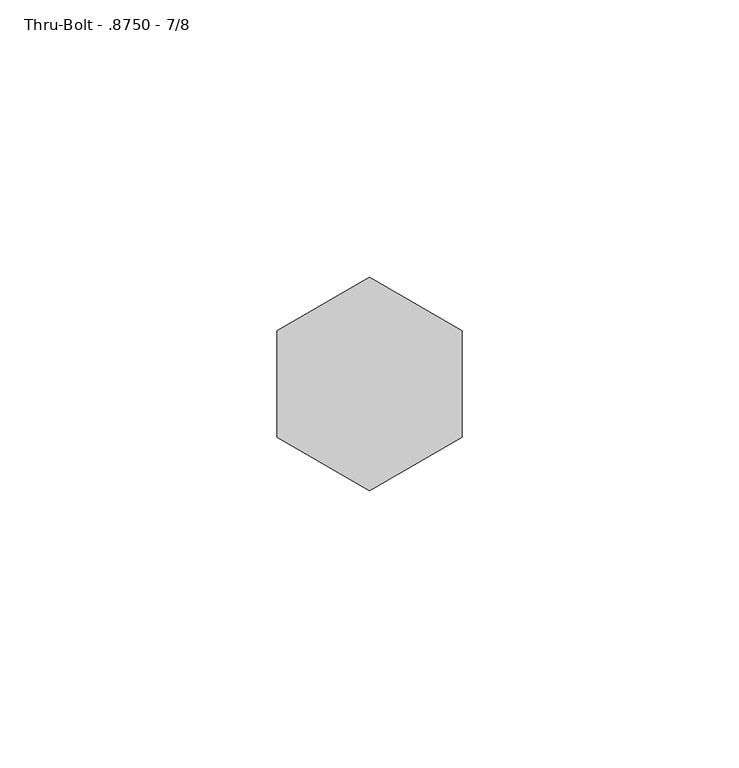
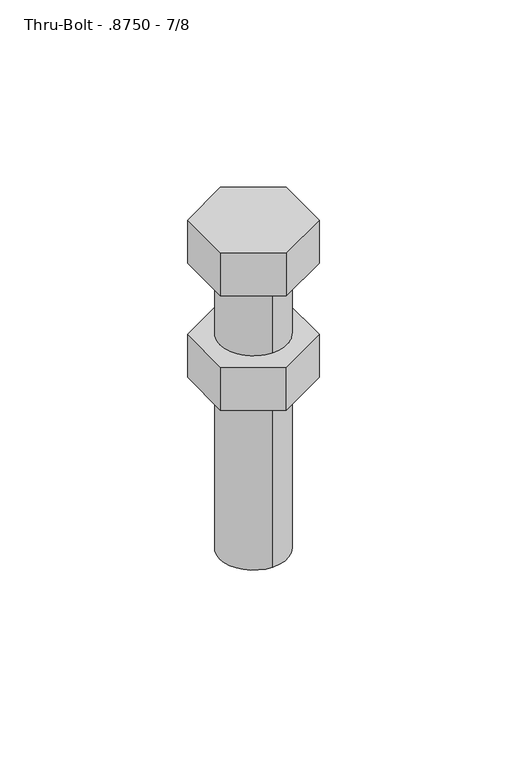
"""IFC4 building model written with IfcOpenShell, lengths in millimetres: fastener geometry, 060523 - W_P_C - Fastenings - Generic : Thru-Bolt - .8750 - 7/8."""

import ifcopenshell
import ifcopenshell.guid

model = None  # the IFC model being written
_history = None  # IfcOwnerHistory: only IFC2X3 demands one
_inside = {}  # id of a spatial element -> (the spatial element, [elements in it])
_under = {}  # id of a project, library or spatial element -> (it, [spatial elements below it])
_declared = {}  # id of a project -> (the project, [libraries it declares])
_typed = {}  # id of a type object -> (the type object, [elements of that type])
_made_of = {}  # id of a material, layer set ... -> (it, [elements and type objects made of it])


def new_model(schema):
    """Start an empty IFC model of exactly this schema.

    Asked for "IFC4X3", IfcOpenShell would pick the latest addendum, in which some entities
    have other attributes; the version numbers below select the first issue.
    IFC2X3 requires an IfcOwnerHistory on every rooted entity: one is made here for all.
    """
    global model, _history
    if schema == "IFC4X3":
        model = ifcopenshell.file(schema_version=(4, 3, 0, 0))
    else:
        model = ifcopenshell.file(schema=schema)
    _inside.clear()
    _under.clear()
    _declared.clear()
    _typed.clear()
    _made_of.clear()
    _history = None
    if model.schema == "IFC2X3":
        org = make("IfcOrganization", Name="unknown")
        user = make(
            "IfcPersonAndOrganization",
            ThePerson=make("IfcPerson", FamilyName="unknown"),
            TheOrganization=org,
        )
        app = make(
            "IfcApplication",
            ApplicationDeveloper=org,
            Version="unknown",
            ApplicationFullName="unknown",
            ApplicationIdentifier="unknown",
        )
        _history = make(
            "IfcOwnerHistory",
            OwningUser=user,
            OwningApplication=app,
            ChangeAction="ADDED",
            CreationDate=0,
        )
    return model


def make(cls, **values):
    """One entity of the class cls with the attributes given. An attribute that is None is left unset."""
    return model.create_entity(
        cls, **{name: value for name, value in values.items() if value is not None}
    )


def rooted(cls, **values):
    """An entity with a GlobalId (a new one), such as an element, a storey or a relation."""
    return make(cls, GlobalId=ifcopenshell.guid.new(), OwnerHistory=_history, **values)


def si_unit(unit_type, name, prefix=None):
    """IfcSIUnit, for example si_unit("LENGTHUNIT", "METRE", prefix="MILLI")."""
    return make("IfcSIUnit", UnitType=unit_type, Prefix=prefix, Name=name)


def assignment(units):
    """IfcUnitAssignment: the units of a project."""
    return None if units is None else make("IfcUnitAssignment", Units=units)


def point(xyz):
    """IfcCartesianPoint."""
    return None if xyz is None else make("IfcCartesianPoint", Coordinates=xyz)


def direction(xyz):
    """IfcDirection."""
    return None if xyz is None else make("IfcDirection", DirectionRatios=xyz)


def frame(location, z_axis=None, x_axis=None):
    """IfcAxis2Placement3D, a coordinate frame: its origin and axes. An axis left out is left unset."""
    return make(
        "IfcAxis2Placement3D",
        Location=point(location),
        Axis=direction(z_axis),
        RefDirection=direction(x_axis),
    )


def frame_2d(location, x_axis=None):
    """IfcAxis2Placement2D, a coordinate frame in the plane: its origin and x axis."""
    return make(
        "IfcAxis2Placement2D", Location=point(location), RefDirection=direction(x_axis)
    )


def origin():
    """The frame at (0, 0, 0) with its axes left unset."""
    return frame((0.0, 0.0, 0.0))


def origin_with_axes():
    """The frame at (0, 0, 0) with the z axis (0, 0, 1) and the x axis (1, 0, 0) written out."""
    return frame((0.0, 0.0, 0.0), z_axis=(0.0, 0.0, 1.0), x_axis=(1.0, 0.0, 0.0))


def origin_2d():
    """The frame at (0, 0) in the plane with its x axis left unset."""
    return frame_2d((0.0, 0.0))


def place(relative_to, where):
    """IfcLocalPlacement: puts the frame where relative to a parent placement (None: the world)."""
    return make(
        "IfcLocalPlacement", PlacementRelTo=relative_to, RelativePlacement=where
    )


def context(
    kind, dimensions, precision=None, world=None, true_north=None, identifier=None
):
    """IfcGeometricRepresentationContext, for example the 3D "Model" context."""
    return make(
        "IfcGeometricRepresentationContext",
        ContextIdentifier=identifier,
        ContextType=kind,
        CoordinateSpaceDimension=dimensions,
        Precision=precision,
        WorldCoordinateSystem=world,
        TrueNorth=true_north,
    )


def project(units=None, contexts=None):
    """IfcProject with its units and contexts."""
    return rooted(
        "IfcProject",
        Name="project",
        RepresentationContexts=contexts,
        UnitsInContext=assignment(units),
    )


def spatial(cls, under=None, at=None, **own):
    """A site, building, storey or space (cls), placed at a placement, below another one or the project."""
    s = rooted(cls, ObjectPlacement=at, **own)
    if under is not None:
        _under.setdefault(under.id(), (under, []))[1].append(s)
    return s


def polyline(points):
    """IfcPolyline through the points."""
    return make("IfcPolyline", Points=[point(p) for p in points])


def circle_curve(where, radius):
    """IfcCircle in the frame where."""
    return make("IfcCircle", Position=where, Radius=radius)


def trimmed(basis, trim1, trim2, sense, master):
    """IfcTrimmedCurve: the piece of a basis curve between two trims."""
    return make(
        "IfcTrimmedCurve",
        BasisCurve=basis,
        Trim1=trim1,
        Trim2=trim2,
        SenseAgreement=sense,
        MasterRepresentation=master,
    )


def segment(curve, same_sense, transition):
    """IfcCompositeCurveSegment."""
    return make(
        "IfcCompositeCurveSegment",
        Transition=transition,
        SameSense=same_sense,
        ParentCurve=curve,
    )


def composite_curve(segments, self_intersect=None):
    """IfcCompositeCurve: segments joined end to end."""
    return make("IfcCompositeCurve", Segments=segments, SelfIntersect=self_intersect)


def outline(outer, holes=None, kind="AREA"):
    """IfcArbitraryClosedProfileDef: a profile drawn as a closed curve; with holes, ...WithVoids."""
    if holes is None:
        return make("IfcArbitraryClosedProfileDef", ProfileType=kind, OuterCurve=outer)
    return make(
        "IfcArbitraryProfileDefWithVoids",
        ProfileType=kind,
        OuterCurve=outer,
        InnerCurves=holes,
    )


def extrude(swept, where, along, depth):
    """IfcExtrudedAreaSolid: the profile swept, set in the frame where, extruded along a direction by depth."""
    return make(
        "IfcExtrudedAreaSolid",
        SweptArea=swept,
        Position=where,
        ExtrudedDirection=direction(along),
        Depth=depth,
    )


def shape(context_of_items, identifier, shape_type, items):
    """IfcShapeRepresentation: the items that make up one representation, for example the "Body"."""
    return make(
        "IfcShapeRepresentation",
        ContextOfItems=context_of_items,
        RepresentationIdentifier=identifier,
        RepresentationType=shape_type,
        Items=items,
    )


def source(mapping_origin, context_of_items, identifier, shape_type, items):
    """IfcRepresentationMap: a shape defined once, which mapped items show again and again."""
    return make(
        "IfcRepresentationMap",
        MappingOrigin=mapping_origin,
        MappedRepresentation=shape(context_of_items, identifier, shape_type, items),
    )


def transform(
    local_origin,
    x_axis=None,
    y_axis=None,
    z_axis=None,
    scale=None,
    scale2=None,
    scale3=None,
    uniform=True,
):
    """IfcCartesianTransformationOperator3D, or its non-uniform kind. x_axis, y_axis, z_axis: its Axis1, 2, 3."""
    if uniform:
        return make(
            "IfcCartesianTransformationOperator3D",
            Axis1=direction(x_axis),
            Axis2=direction(y_axis),
            LocalOrigin=point(local_origin),
            Scale=scale,
            Axis3=direction(z_axis),
        )
    return make(
        "IfcCartesianTransformationOperator3DnonUniform",
        Axis1=direction(x_axis),
        Axis2=direction(y_axis),
        LocalOrigin=point(local_origin),
        Scale=scale,
        Axis3=direction(z_axis),
        Scale2=scale2,
        Scale3=scale3,
    )


def mapped(mapping_source, mapping_target):
    """IfcMappedItem: shows the shape of a source again, moved by a transform."""
    return make(
        "IfcMappedItem", MappingSource=mapping_source, MappingTarget=mapping_target
    )


def made_of(thing, what):
    """Note that an element or type object is made of a material, layer set ...; save() writes the relation."""
    if what is not None:
        _made_of.setdefault(what.id(), (what, []))[1].append(thing)
    return thing


def element(
    cls,
    number,
    at=None,
    inside=None,
    cuts=None,
    type_object=None,
    material=None,
    context=None,
    identifier="Body",
    shape_type=None,
    held_by="IfcProductDefinitionShape",
    body=None,
    shapes=None,
    **own,
):
    """One element of the class cls, such as IfcWall. Its Tag is "e" and its number.

    at: its placement. inside: the storey or other place that contains it. cuts: it is an
    opening in that element (IfcRelVoidsElement). A single representation is given by context,
    identifier, shape_type and body (its items); several are given by shapes. held_by: the class
    of the entity that holds the representations. save() writes the other relations.
    """
    e = rooted(cls, Tag="e%d" % number, ObjectPlacement=at, **own)
    if body is not None:
        shapes = [shape(context, identifier, shape_type, body)]
    if shapes is not None:
        e.Representation = make(held_by, Representations=shapes)
    if inside is not None:
        _inside.setdefault(inside.id(), (inside, []))[1].append(e)
    if cuts is not None:
        rooted(
            "IfcRelVoidsElement", RelatingBuildingElement=cuts, RelatedOpeningElement=e
        )
    if type_object is not None:
        _typed.setdefault(type_object.id(), (type_object, []))[1].append(e)
    return made_of(e, material)


def aggregate(whole, parts):
    """IfcRelAggregates: a whole, such as a stair, and the parts it consists of."""
    return rooted("IfcRelAggregates", RelatingObject=whole, RelatedObjects=parts)


def save(model, path):
    """Write the relations noted so far, then the file.

    IfcRelAggregates (storeys below a building ...), IfcRelContainedInSpatialStructure (elements
    in a storey), IfcRelDefinesByType, IfcRelAssociatesMaterial and IfcRelDeclares: one each for
    every whole, place, type object, material and project.
    """
    for whole, parts in _under.values():
        aggregate(whole, parts)
    for where, things in _inside.values():
        rooted(
            "IfcRelContainedInSpatialStructure",
            RelatedElements=things,
            RelatingStructure=where,
        )
    for kind, things in _typed.values():
        rooted("IfcRelDefinesByType", RelatedObjects=things, RelatingType=kind)
    for what, things in _made_of.values():
        rooted("IfcRelAssociatesMaterial", RelatedObjects=things, RelatingMaterial=what)
    for by, libraries in _declared.values():
        rooted("IfcRelDeclares", RelatingContext=by, RelatedDefinitions=libraries)
    model.write(path)


def thru_bolt_8750_7_8_fa354763(model_context):
    return source(origin(), model_context, "Body", "SweptSolid", [
        extrude(outline(polyline([(-16.66875, -9.6237073), (-16.66875, 9.6237073), (0.0, 19.2474146), (16.66875, 9.6237073), (16.66875, -9.6237073), (0.0, -19.2474146), (-16.66875, -9.6237073)])), frame((0.0, 0.0, -40.7789063), z_axis=(0.0, 0.0, 1.0), x_axis=(1.0, 0.0, 0.0)), (0.0, 0.0, 1.0), 15.3789062),
        extrude(outline(polyline([(-16.66875, 9.6237073), (0.0, 19.2474146), (16.66875, 9.6237073), (16.66875, -9.6237073), (0.0, -19.2474146), (-16.66875, -9.6237073), (-16.66875, 9.6237073)])), origin_with_axes(), (0.0, 0.0, 1.0), 15.3789062),
        extrude(outline(composite_curve([segment(trimmed(circle_curve(origin_2d(), 11.3605469), [point((0.0, -11.3605469))], [point((0.0, 11.3605469))], False, "CARTESIAN"), True, "CONTINUOUS"), segment(trimmed(circle_curve(origin_2d(), 11.3605469), [point((0.0, 11.3605469))], [point((0.0, -11.3605469))], False, "CARTESIAN"), True, "CONTINUOUS")], self_intersect=False)), frame((0.0, 0.0, -101.6), z_axis=(0.0, 0.0, 1.0), x_axis=(1.0, 0.0, 0.0)), (0.0, 0.0, 1.0), 101.6),
    ])


if __name__ == "__main__":
    model = new_model("IFC4")
    model_context = context("Model", 3, world=origin())
    ifc_project = project(units=[si_unit("LENGTHUNIT", "METRE", prefix="MILLI")], contexts=[model_context])
    site = spatial("IfcSite", under=ifc_project)
    building = spatial("IfcBuilding", under=site)
    placement = place(None, origin())
    thru_bolt_8750_7_8_shape = thru_bolt_8750_7_8_fa354763(model_context)
    element("IfcFastener", 1, ObjectType="060523 - W_P_C - Fastenings - Generic : Thru-Bolt - .8750 - 7/8", at=placement, inside=building, context=model_context, shape_type="MappedRepresentation", body=[
        mapped(thru_bolt_8750_7_8_shape, transform((0.0, 0.0, 0.0), x_axis=(1.0, 0.0, 0.0), y_axis=(0.0, 1.0, 0.0), z_axis=(0.0, 0.0, 1.0))),
    ])
    save(model, "model.ifc")

# Revit data of these elements
# Type "060523 - W_P_C - Fastenings - Generic : Thru-Bolt - .8750 - 7/8"
#   Washer_Thickness = 0' - 0.20182"
#   Washer Radius = 0' - 1.05273"
#   Washer Offset - Head = 0' - 0"
#   Washer Offset = 0' - 0"
#   Thickness_of_Substrate [instance default] = 0' - 1"
#   Side = 0' - 0.75879"
#   Radius = 0' - 0.44727"
#   Length [instance default] = 0' - 4"
#   Head Size = 0' - 1 5/16"
#   Head Radius = 0' - 0 21/32"
#   Head Height = 0' - 0 155/256"
#   Double Diameter = 0' - 1 101/128"
#   Diameter = 0' - 0 229/256"
#   Default Elevation = 4' - 0"
#   Washer_Nut_Visibility = no
#   Washer_Head_Visibility = no
#   Round_Head_Visibility = no
#   Point Visibility = no
#   Nut_Visibility = yes
#   Hex_Head_Visiblilty = yes
#   Washer Material = none
#   Bolt Material (Size) = AT SILL - FASTENER AT 24" O.C.
# Element 1 (IfcFastener, "060523 - W_P_C - Fastenings - Generic : Thru-Bolt - .8750 - 7/8")
#   Materials on its faces: "AT SILL - FASTENER AT 24\" O.C."
# Materials
#   "AT SILL - FASTENER AT 24\" O.C.": class "Generic", colour RGB 120 120 120, transparency 0, Cost = 0
